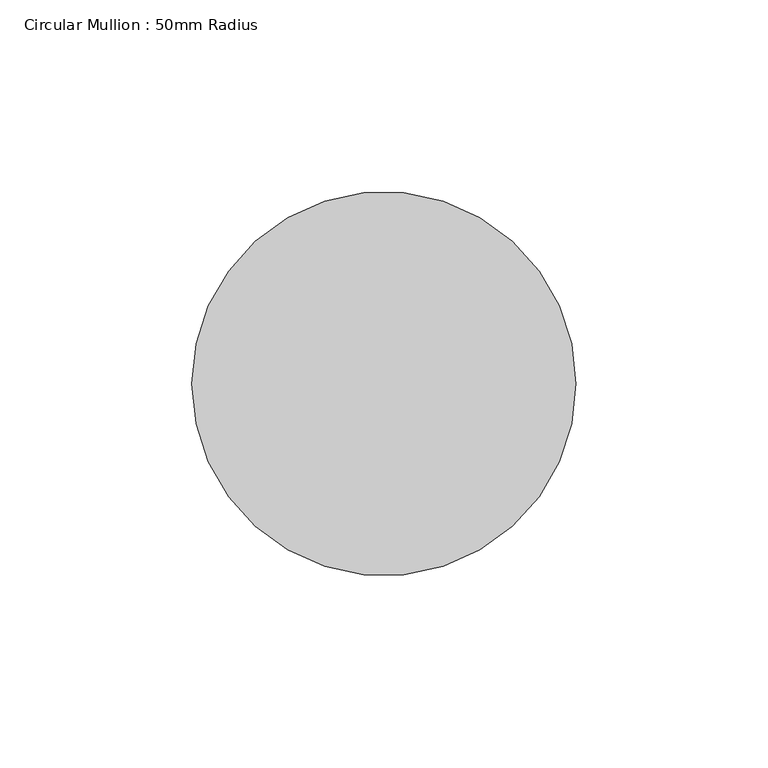
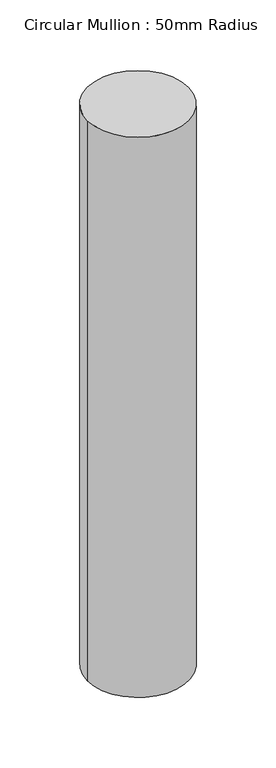
"""IFC4 building model written with IfcOpenShell, lengths in millimetres: member geometry, Circular Mullion : 50mm Radius."""

from ifc_helpers import new_model, si_unit, point, frame, origin, origin_2d, place, context, project, spatial, circle_curve, trimmed, segment, composite_curve, outline, extrude, source, transform, mapped, element, save


def circular_mullion_50mm_radius_2b4f3948(model_context):
    return source(origin(), model_context, "Body", "SweptSolid", [
        extrude(outline(composite_curve([segment(trimmed(circle_curve(origin_2d(), 50.0), [point((50.0, 0.0))], [point((-50.0, 0.0))], False, "CARTESIAN"), True, "CONTINUOUS"), segment(trimmed(circle_curve(origin_2d(), 50.0), [point((-50.0, 0.0))], [point((50.0, 0.0))], False, "CARTESIAN"), True, "CONTINUOUS")], self_intersect=False)), frame((0.0, 0.0, -586.6958873), z_axis=(0.0, 0.0, 1.0), x_axis=(1.0, 0.0, 0.0)), (0.0, 0.0, 1.0), 586.6958873),
    ])


if __name__ == "__main__":
    model = new_model("IFC4")
    model_context = context("Model", 3, world=origin())
    ifc_project = project(units=[si_unit("LENGTHUNIT", "METRE", prefix="MILLI")], contexts=[model_context])
    site = spatial("IfcSite", under=ifc_project)
    building = spatial("IfcBuilding", under=site)
    placement = place(None, origin())
    circular_mullion_50mm_radius_shape = circular_mullion_50mm_radius_2b4f3948(model_context)
    element("IfcMember", 1, ObjectType="Circular Mullion : 50mm Radius", at=placement, inside=building, context=model_context, shape_type="MappedRepresentation", body=[
        mapped(circular_mullion_50mm_radius_shape, transform((0.0, 0.0, 0.0), x_axis=(1.0, 0.0, 0.0), y_axis=(0.0, 1.0, 0.0), z_axis=(0.0, 0.0, 1.0))),
    ])
    save(model, "model.ifc")

# Revit data of these elements
# Type "Circular Mullion : 50mm Radius"
#   built-in parameter 1007350 = 0.164042 (stored number, unit not read)
# Element 1 (IfcMember, "Circular Mullion : 50mm Radius")
#   Materials on its faces: "Aluminium"
# Materials
#   "Aluminium": class "Metal", colour RGB 247 247 247, transparency 0, Description = "Aluminium 6061", Cost = 0
